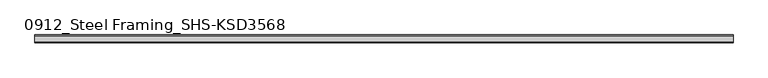
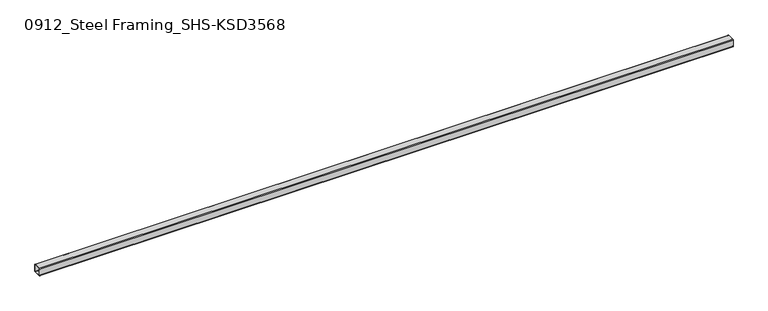
"""IFC4 building model written with IfcOpenShell, lengths in millimetres: beam geometry, 0912_Steel Framing_SHS-KSD3568 : H_SB_ASB_SHS-150x150x6."""

from ifc_helpers import new_model, si_unit, point, frame, frame_2d, origin, place, context, project, spatial, polyline, circle_curve, trimmed, segment, composite_curve, outline, extrude, source, transform, mapped, element, save


def beam_0912_steel_framing_shs_ksd3568_6ae5eb3c(model_context):
    return source(origin(), model_context, "Body", "SweptSolid", [
        extrude(outline(composite_curve([segment(polyline([(75.0, 63.0), (75.0, -63.0)]), True, "CONTINUOUS"), segment(trimmed(circle_curve(frame_2d((63.0, -63.0)), 12.0), [point((75.0, -63.0))], [point((63.0, -75.0))], False, "CARTESIAN"), True, "CONTINUOUS"), segment(polyline([(63.0, -75.0), (-63.0, -75.0)]), True, "CONTINUOUS"), segment(trimmed(circle_curve(frame_2d((-63.0, -63.0)), 12.0), [point((-63.0, -75.0))], [point((-75.0, -63.0))], False, "CARTESIAN"), True, "CONTINUOUS"), segment(polyline([(-75.0, -63.0), (-75.0, 63.0)]), True, "CONTINUOUS"), segment(trimmed(circle_curve(frame_2d((-63.0, 63.0)), 12.0), [point((-75.0, 63.0))], [point((-63.0, 75.0))], False, "CARTESIAN"), True, "CONTINUOUS"), segment(polyline([(-63.0, 75.0), (63.0, 75.0)]), True, "CONTINUOUS"), segment(trimmed(circle_curve(frame_2d((63.0, 63.0)), 12.0), [point((63.0, 75.0))], [point((75.0, 63.0))], False, "CARTESIAN"), True, "CONTINUOUS")], self_intersect=False), holes=[composite_curve([segment(trimmed(circle_curve(frame_2d((-63.0, 63.0)), 6.0), [point((-63.0, 69.0))], [point((-69.0, 63.0))], True, "CARTESIAN"), True, "CONTINUOUS"), segment(polyline([(-69.0, 63.0), (-69.0, -63.0)]), True, "CONTINUOUS"), segment(trimmed(circle_curve(frame_2d((-63.0, -63.0)), 6.0), [point((-69.0, -63.0))], [point((-63.0, -69.0))], True, "CARTESIAN"), True, "CONTINUOUS"), segment(polyline([(-63.0, -69.0), (63.0, -69.0)]), True, "CONTINUOUS"), segment(trimmed(circle_curve(frame_2d((63.0, -63.0)), 6.0), [point((63.0, -69.0))], [point((69.0, -63.0))], True, "CARTESIAN"), True, "CONTINUOUS"), segment(polyline([(69.0, -63.0), (69.0, 63.0)]), True, "CONTINUOUS"), segment(trimmed(circle_curve(frame_2d((63.0, 63.0)), 6.0), [point((69.0, 63.0))], [point((63.0, 69.0))], True, "CARTESIAN"), True, "CONTINUOUS"), segment(polyline([(63.0, 69.0), (-63.0, 69.0)]), True, "CONTINUOUS")], self_intersect=False)]), frame((-6620.9, 0.0, 0.0), z_axis=(1.0, 0.0, 0.0), x_axis=(0.0, 1.0, 0.0)), (0.0, 0.0, 1.0), 13241.8),
    ])


if __name__ == "__main__":
    model = new_model("IFC4")
    model_context = context("Model", 3, world=origin())
    ifc_project = project(units=[si_unit("LENGTHUNIT", "METRE", prefix="MILLI")], contexts=[model_context])
    site = spatial("IfcSite", under=ifc_project)
    building = spatial("IfcBuilding", under=site)
    placement = place(None, origin())
    beam_0912_steel_framing_shs_ksd3568_shape = beam_0912_steel_framing_shs_ksd3568_6ae5eb3c(model_context)
    element("IfcBeam", 1, ObjectType="0912_Steel Framing_SHS-KSD3568 : H_SB_ASB_SHS-150x150x6", at=placement, inside=building, context=model_context, shape_type="MappedRepresentation", body=[
        mapped(beam_0912_steel_framing_shs_ksd3568_shape, transform((0.0, 0.0, 0.0), x_axis=(1.0, 0.0, 0.0), y_axis=(0.0, 1.0, 0.0), z_axis=(0.0, 0.0, 1.0))),
    ])
    save(model, "model.ifc")

# Revit data of these elements
# Type "0912_Steel Framing_SHS-KSD3568 : H_SB_ASB_SHS-150x150x6"
#   H_WM Code_1 = "S01AA002-00001 | Main Steel Structure Fabrication Work | Shelter/Building | Medium Steel - Standard (90KG/M>Weight≥30KG/M) | Material: (   )"
#   H_WM Code_2 = "S03AA028-00001 | Main Steel Structure Erection Work | Shelter/Building | Medium Steel (90KG/M>Weight≥30KG/M) | Material: (   )"
#   H_WM Code_3 = "S01AA010-00001 | Main Steel Structure Fabrication Work | Shelter/Building | Steel Painting/Coating | for Non-Fireproofed Steel Surface, Surface Preparation, Primer, Second & Final Coat | Material: (   )"
#   H_Q'ty Cal Type Tag = "SB-Q2"
#   Perimeter = 0.60 m²/m
#   Nominal Weight = 26.40 kgf/m
#   Length [instance default] = 1.0000 m
#   b = 0.1500 m
#   h = 0.1500 m
#   tr = 0.0120 m
#   t = 0.0060 m
#   A = 28.36 m²
#   Structural Material [instance default] = Steel, 45-345
# Element 1 (IfcBeam, "0912_Steel Framing_SHS-KSD3568 : H_SB_ASB_SHS-150x150x6")
#   Structural Material = none
# Materials
#   "Steel, 45-345": class "Metal", colour RGB 189 187 185, transparency 0, Description = "Steel 345 MPa", Cost = 0
